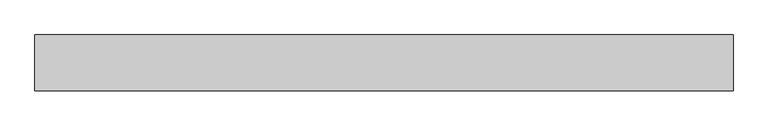
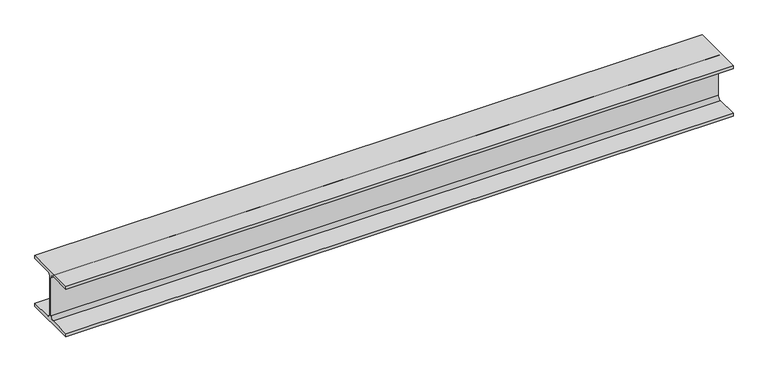
"""IFC4 building model written with IfcOpenShell, lengths in millimetres: beam geometry, 0912_Steel Framing_H-KSD3502 : H_SB_ASB_H-200x200x8x12."""

import ifcopenshell
import ifcopenshell.guid

model = None  # the IFC model being written
_history = None  # IfcOwnerHistory: only IFC2X3 demands one
_inside = {}  # id of a spatial element -> (the spatial element, [elements in it])
_under = {}  # id of a project, library or spatial element -> (it, [spatial elements below it])
_declared = {}  # id of a project -> (the project, [libraries it declares])
_typed = {}  # id of a type object -> (the type object, [elements of that type])
_made_of = {}  # id of a material, layer set ... -> (it, [elements and type objects made of it])


def new_model(schema):
    """Start an empty IFC model of exactly this schema.

    Asked for "IFC4X3", IfcOpenShell would pick the latest addendum, in which some entities
    have other attributes; the version numbers below select the first issue.
    IFC2X3 requires an IfcOwnerHistory on every rooted entity: one is made here for all.
    """
    global model, _history
    if schema == "IFC4X3":
        model = ifcopenshell.file(schema_version=(4, 3, 0, 0))
    else:
        model = ifcopenshell.file(schema=schema)
    _inside.clear()
    _under.clear()
    _declared.clear()
    _typed.clear()
    _made_of.clear()
    _history = None
    if model.schema == "IFC2X3":
        org = make("IfcOrganization", Name="unknown")
        user = make(
            "IfcPersonAndOrganization",
            ThePerson=make("IfcPerson", FamilyName="unknown"),
            TheOrganization=org,
        )
        app = make(
            "IfcApplication",
            ApplicationDeveloper=org,
            Version="unknown",
            ApplicationFullName="unknown",
            ApplicationIdentifier="unknown",
        )
        _history = make(
            "IfcOwnerHistory",
            OwningUser=user,
            OwningApplication=app,
            ChangeAction="ADDED",
            CreationDate=0,
        )
    return model


def make(cls, **values):
    """One entity of the class cls with the attributes given. An attribute that is None is left unset."""
    return model.create_entity(
        cls, **{name: value for name, value in values.items() if value is not None}
    )


def rooted(cls, **values):
    """An entity with a GlobalId (a new one), such as an element, a storey or a relation."""
    return make(cls, GlobalId=ifcopenshell.guid.new(), OwnerHistory=_history, **values)


def si_unit(unit_type, name, prefix=None):
    """IfcSIUnit, for example si_unit("LENGTHUNIT", "METRE", prefix="MILLI")."""
    return make("IfcSIUnit", UnitType=unit_type, Prefix=prefix, Name=name)


def assignment(units):
    """IfcUnitAssignment: the units of a project."""
    return None if units is None else make("IfcUnitAssignment", Units=units)


def point(xyz):
    """IfcCartesianPoint."""
    return None if xyz is None else make("IfcCartesianPoint", Coordinates=xyz)


def direction(xyz):
    """IfcDirection."""
    return None if xyz is None else make("IfcDirection", DirectionRatios=xyz)


def frame(location, z_axis=None, x_axis=None):
    """IfcAxis2Placement3D, a coordinate frame: its origin and axes. An axis left out is left unset."""
    return make(
        "IfcAxis2Placement3D",
        Location=point(location),
        Axis=direction(z_axis),
        RefDirection=direction(x_axis),
    )


def frame_2d(location, x_axis=None):
    """IfcAxis2Placement2D, a coordinate frame in the plane: its origin and x axis."""
    return make(
        "IfcAxis2Placement2D", Location=point(location), RefDirection=direction(x_axis)
    )


def origin():
    """The frame at (0, 0, 0) with its axes left unset."""
    return frame((0.0, 0.0, 0.0))


def place(relative_to, where):
    """IfcLocalPlacement: puts the frame where relative to a parent placement (None: the world)."""
    return make(
        "IfcLocalPlacement", PlacementRelTo=relative_to, RelativePlacement=where
    )


def context(
    kind, dimensions, precision=None, world=None, true_north=None, identifier=None
):
    """IfcGeometricRepresentationContext, for example the 3D "Model" context."""
    return make(
        "IfcGeometricRepresentationContext",
        ContextIdentifier=identifier,
        ContextType=kind,
        CoordinateSpaceDimension=dimensions,
        Precision=precision,
        WorldCoordinateSystem=world,
        TrueNorth=true_north,
    )


def project(units=None, contexts=None):
    """IfcProject with its units and contexts."""
    return rooted(
        "IfcProject",
        Name="project",
        RepresentationContexts=contexts,
        UnitsInContext=assignment(units),
    )


def spatial(cls, under=None, at=None, **own):
    """A site, building, storey or space (cls), placed at a placement, below another one or the project."""
    s = rooted(cls, ObjectPlacement=at, **own)
    if under is not None:
        _under.setdefault(under.id(), (under, []))[1].append(s)
    return s


def polyline(points):
    """IfcPolyline through the points."""
    return make("IfcPolyline", Points=[point(p) for p in points])


def circle_curve(where, radius):
    """IfcCircle in the frame where."""
    return make("IfcCircle", Position=where, Radius=radius)


def trimmed(basis, trim1, trim2, sense, master):
    """IfcTrimmedCurve: the piece of a basis curve between two trims."""
    return make(
        "IfcTrimmedCurve",
        BasisCurve=basis,
        Trim1=trim1,
        Trim2=trim2,
        SenseAgreement=sense,
        MasterRepresentation=master,
    )


def segment(curve, same_sense, transition):
    """IfcCompositeCurveSegment."""
    return make(
        "IfcCompositeCurveSegment",
        Transition=transition,
        SameSense=same_sense,
        ParentCurve=curve,
    )


def composite_curve(segments, self_intersect=None):
    """IfcCompositeCurve: segments joined end to end."""
    return make("IfcCompositeCurve", Segments=segments, SelfIntersect=self_intersect)


def outline(outer, holes=None, kind="AREA"):
    """IfcArbitraryClosedProfileDef: a profile drawn as a closed curve; with holes, ...WithVoids."""
    if holes is None:
        return make("IfcArbitraryClosedProfileDef", ProfileType=kind, OuterCurve=outer)
    return make(
        "IfcArbitraryProfileDefWithVoids",
        ProfileType=kind,
        OuterCurve=outer,
        InnerCurves=holes,
    )


def extrude(swept, where, along, depth):
    """IfcExtrudedAreaSolid: the profile swept, set in the frame where, extruded along a direction by depth."""
    return make(
        "IfcExtrudedAreaSolid",
        SweptArea=swept,
        Position=where,
        ExtrudedDirection=direction(along),
        Depth=depth,
    )


def shape(context_of_items, identifier, shape_type, items):
    """IfcShapeRepresentation: the items that make up one representation, for example the "Body"."""
    return make(
        "IfcShapeRepresentation",
        ContextOfItems=context_of_items,
        RepresentationIdentifier=identifier,
        RepresentationType=shape_type,
        Items=items,
    )


def source(mapping_origin, context_of_items, identifier, shape_type, items):
    """IfcRepresentationMap: a shape defined once, which mapped items show again and again."""
    return make(
        "IfcRepresentationMap",
        MappingOrigin=mapping_origin,
        MappedRepresentation=shape(context_of_items, identifier, shape_type, items),
    )


def transform(
    local_origin,
    x_axis=None,
    y_axis=None,
    z_axis=None,
    scale=None,
    scale2=None,
    scale3=None,
    uniform=True,
):
    """IfcCartesianTransformationOperator3D, or its non-uniform kind. x_axis, y_axis, z_axis: its Axis1, 2, 3."""
    if uniform:
        return make(
            "IfcCartesianTransformationOperator3D",
            Axis1=direction(x_axis),
            Axis2=direction(y_axis),
            LocalOrigin=point(local_origin),
            Scale=scale,
            Axis3=direction(z_axis),
        )
    return make(
        "IfcCartesianTransformationOperator3DnonUniform",
        Axis1=direction(x_axis),
        Axis2=direction(y_axis),
        LocalOrigin=point(local_origin),
        Scale=scale,
        Axis3=direction(z_axis),
        Scale2=scale2,
        Scale3=scale3,
    )


def mapped(mapping_source, mapping_target):
    """IfcMappedItem: shows the shape of a source again, moved by a transform."""
    return make(
        "IfcMappedItem", MappingSource=mapping_source, MappingTarget=mapping_target
    )


def made_of(thing, what):
    """Note that an element or type object is made of a material, layer set ...; save() writes the relation."""
    if what is not None:
        _made_of.setdefault(what.id(), (what, []))[1].append(thing)
    return thing


def element(
    cls,
    number,
    at=None,
    inside=None,
    cuts=None,
    type_object=None,
    material=None,
    context=None,
    identifier="Body",
    shape_type=None,
    held_by="IfcProductDefinitionShape",
    body=None,
    shapes=None,
    **own,
):
    """One element of the class cls, such as IfcWall. Its Tag is "e" and its number.

    at: its placement. inside: the storey or other place that contains it. cuts: it is an
    opening in that element (IfcRelVoidsElement). A single representation is given by context,
    identifier, shape_type and body (its items); several are given by shapes. held_by: the class
    of the entity that holds the representations. save() writes the other relations.
    """
    e = rooted(cls, Tag="e%d" % number, ObjectPlacement=at, **own)
    if body is not None:
        shapes = [shape(context, identifier, shape_type, body)]
    if shapes is not None:
        e.Representation = make(held_by, Representations=shapes)
    if inside is not None:
        _inside.setdefault(inside.id(), (inside, []))[1].append(e)
    if cuts is not None:
        rooted(
            "IfcRelVoidsElement", RelatingBuildingElement=cuts, RelatedOpeningElement=e
        )
    if type_object is not None:
        _typed.setdefault(type_object.id(), (type_object, []))[1].append(e)
    return made_of(e, material)


def aggregate(whole, parts):
    """IfcRelAggregates: a whole, such as a stair, and the parts it consists of."""
    return rooted("IfcRelAggregates", RelatingObject=whole, RelatedObjects=parts)


def save(model, path):
    """Write the relations noted so far, then the file.

    IfcRelAggregates (storeys below a building ...), IfcRelContainedInSpatialStructure (elements
    in a storey), IfcRelDefinesByType, IfcRelAssociatesMaterial and IfcRelDeclares: one each for
    every whole, place, type object, material and project.
    """
    for whole, parts in _under.values():
        aggregate(whole, parts)
    for where, things in _inside.values():
        rooted(
            "IfcRelContainedInSpatialStructure",
            RelatedElements=things,
            RelatingStructure=where,
        )
    for kind, things in _typed.values():
        rooted("IfcRelDefinesByType", RelatedObjects=things, RelatingType=kind)
    for what, things in _made_of.values():
        rooted("IfcRelAssociatesMaterial", RelatedObjects=things, RelatingMaterial=what)
    for by, libraries in _declared.values():
        rooted("IfcRelDeclares", RelatingContext=by, RelatedDefinitions=libraries)
    model.write(path)


def beam_1d2e41cb(model_context):
    return source(origin(), model_context, "Body", "SweptSolid", [
        extrude(outline(composite_curve([segment(polyline([(100.0, -88.0), (100.0, -100.0), (-100.0, -100.0), (-100.0, -88.0), (-17.0, -88.0)]), True, "CONTINUOUS"), segment(trimmed(circle_curve(frame_2d((-17.0, -75.0)), 13.0), [point((-17.0, -88.0))], [point((-4.0, -75.0))], True, "CARTESIAN"), True, "CONTINUOUS"), segment(polyline([(-4.0, -75.0), (-4.0, 75.0)]), True, "CONTINUOUS"), segment(trimmed(circle_curve(frame_2d((-17.0, 75.0)), 13.0), [point((-4.0, 75.0))], [point((-17.0, 88.0))], True, "CARTESIAN"), True, "CONTINUOUS"), segment(polyline([(-17.0, 88.0), (-100.0, 88.0), (-100.0, 100.0), (100.0, 100.0), (100.0, 88.0), (17.0, 88.0)]), True, "CONTINUOUS"), segment(trimmed(circle_curve(frame_2d((17.0, 75.0)), 13.0), [point((17.0, 88.0))], [point((4.0, 75.0))], True, "CARTESIAN"), True, "CONTINUOUS"), segment(polyline([(4.0, 75.0), (4.0, -75.0)]), True, "CONTINUOUS"), segment(trimmed(circle_curve(frame_2d((17.0, -75.0)), 13.0), [point((4.0, -75.0))], [point((17.0, -88.0))], True, "CARTESIAN"), True, "CONTINUOUS"), segment(polyline([(17.0, -88.0), (100.0, -88.0)]), True, "CONTINUOUS")], self_intersect=False)), frame((-1270.5762137, 0.0, 0.0), z_axis=(1.0, 0.0, 0.0), x_axis=(0.0, 1.0, 0.0)), (0.0, 0.0, 1.0), 2490.6760125),
    ])


if __name__ == "__main__":
    model = new_model("IFC4")
    model_context = context("Model", 3, world=origin())
    ifc_project = project(units=[si_unit("LENGTHUNIT", "METRE", prefix="MILLI")], contexts=[model_context])
    site = spatial("IfcSite", under=ifc_project)
    building = spatial("IfcBuilding", under=site)
    placement = place(None, origin())
    beam_shape = beam_1d2e41cb(model_context)
    element("IfcBeam", 1, ObjectType="0912_Steel Framing_H-KSD3502 : H_SB_ASB_H-200x200x8x12", at=placement, inside=building, context=model_context, shape_type="MappedRepresentation", body=[
        mapped(beam_shape, transform((0.0, 0.0, 0.0), x_axis=(1.0, 0.0, 0.0), y_axis=(0.0, 1.0, 0.0), z_axis=(0.0, 0.0, 1.0))),
    ])
    save(model, "model.ifc")

# Revit data of these elements
# Type "0912_Steel Framing_H-KSD3502 : H_SB_ASB_H-200x200x8x12"
#   H_WM Code_1 = "S01AA002-00001 | Main Steel Structure Fabrication Work | Shelter/Building | Medium Steel - Standard (90KG/M>Weight≥30KG/M) | Material: (   )"
#   H_WM Code_2 = "S03AA028-00001 | Main Steel Structure Erection Work | Shelter/Building | Medium Steel (90KG/M>Weight≥30KG/M) | Material: (   )"
#   H_WM Code_3 = "S01AA010-00001 | Main Steel Structure Fabrication Work | Shelter/Building | Steel Painting/Coating | for Non-Fireproofed Steel Surface, Surface Preparation, Primer, Second & Final Coat | Material: (   )"
#   H_Q'ty Cal Type Tag = "SB-Q2"
#   Width = 20.0 cm
#   Web Thickness = 0.8 cm
#   Web Fillet = 1.3 cm
#   Warping Constant = 141000.0 cm⁶
#   W = 0
#   Torsional Moment of Inertia = 26.2485 cm⁴
#   Section Area = 63.53 cm²
#   Plastic Modulus weak axis = 244.0 cm³
#   Plastic Modulus strong axis = 525.0 cm³
#   Perimeter = 1.16 m²/m
#   Nominal Weight = 49.90 kgf/m
#   Moment of Inertia weak axis = 1600.00 cm⁴
#   Moment of Inertia strong axis = 4720.00 cm⁴
#   Height = 20.0 cm
#   Flange Thickness = 1.2 cm
#   Elastic Modulus weak axis = 160.0 cm³
#   Elastic Modulus strong axis = 472.0 cm³
#   Centroid Vertical = 10.0 cm
#   Centroid Horizontal = 10.0 cm
#   Ix = 47200000
#   Length [instance default] = 1.5240 m
#   Zx = 525000
#   b = 0.2000 m
#   h = 0.2000 m
#   r = 0.0130 m
#   s = 0.0080 m
#   t = 0.0120 m
#   A = 0.006353 m²
#   Structural Material [instance default] = Steel, 45-345
#   Assembly Code = ""
# Element 1 (IfcBeam, "0912_Steel Framing_H-KSD3502 : H_SB_ASB_H-200x200x8x12")
#   Structural Material = none
# Materials
#   "Steel, 45-345": class "Metal", colour RGB 189 187 185, transparency 0, Description = "Steel 345 MPa", Cost = 0
